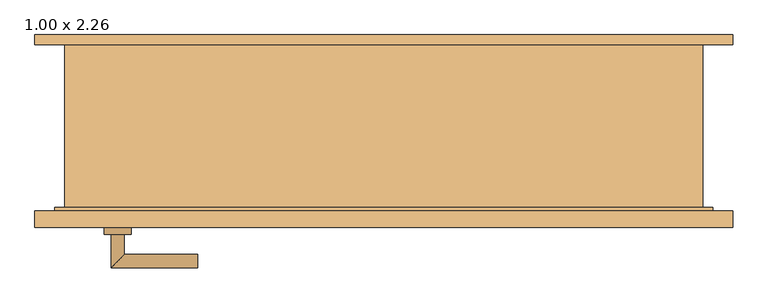
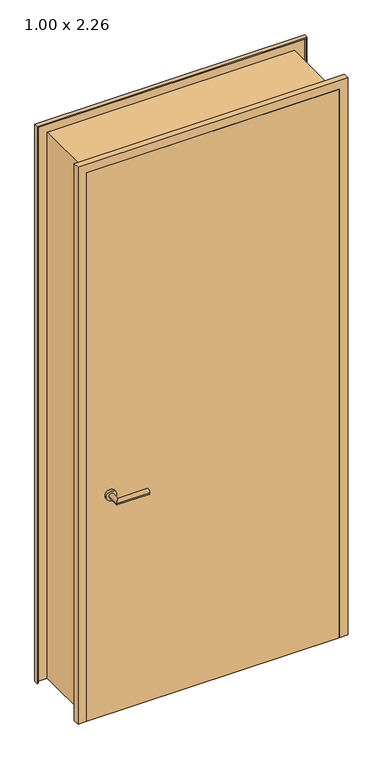
"""IFC4 building model written with IfcOpenShell, lengths in millimetres: door geometry, Drehflügel 1-flg - Stahlzarge : 1.00 x 2.26."""

import ifcopenshell
import ifcopenshell.guid

model = None  # the IFC model being written
_history = None  # IfcOwnerHistory: only IFC2X3 demands one
_inside = {}  # id of a spatial element -> (the spatial element, [elements in it])
_under = {}  # id of a project, library or spatial element -> (it, [spatial elements below it])
_declared = {}  # id of a project -> (the project, [libraries it declares])
_typed = {}  # id of a type object -> (the type object, [elements of that type])
_made_of = {}  # id of a material, layer set ... -> (it, [elements and type objects made of it])


def new_model(schema):
    """Start an empty IFC model of exactly this schema.

    Asked for "IFC4X3", IfcOpenShell would pick the latest addendum, in which some entities
    have other attributes; the version numbers below select the first issue.
    IFC2X3 requires an IfcOwnerHistory on every rooted entity: one is made here for all.
    """
    global model, _history
    if schema == "IFC4X3":
        model = ifcopenshell.file(schema_version=(4, 3, 0, 0))
    else:
        model = ifcopenshell.file(schema=schema)
    _inside.clear()
    _under.clear()
    _declared.clear()
    _typed.clear()
    _made_of.clear()
    _history = None
    if model.schema == "IFC2X3":
        org = make("IfcOrganization", Name="unknown")
        user = make(
            "IfcPersonAndOrganization",
            ThePerson=make("IfcPerson", FamilyName="unknown"),
            TheOrganization=org,
        )
        app = make(
            "IfcApplication",
            ApplicationDeveloper=org,
            Version="unknown",
            ApplicationFullName="unknown",
            ApplicationIdentifier="unknown",
        )
        _history = make(
            "IfcOwnerHistory",
            OwningUser=user,
            OwningApplication=app,
            ChangeAction="ADDED",
            CreationDate=0,
        )
    return model


def make(cls, **values):
    """One entity of the class cls with the attributes given. An attribute that is None is left unset."""
    return model.create_entity(
        cls, **{name: value for name, value in values.items() if value is not None}
    )


def rooted(cls, **values):
    """An entity with a GlobalId (a new one), such as an element, a storey or a relation."""
    return make(cls, GlobalId=ifcopenshell.guid.new(), OwnerHistory=_history, **values)


def si_unit(unit_type, name, prefix=None):
    """IfcSIUnit, for example si_unit("LENGTHUNIT", "METRE", prefix="MILLI")."""
    return make("IfcSIUnit", UnitType=unit_type, Prefix=prefix, Name=name)


def assignment(units):
    """IfcUnitAssignment: the units of a project."""
    return None if units is None else make("IfcUnitAssignment", Units=units)


def point(xyz):
    """IfcCartesianPoint."""
    return None if xyz is None else make("IfcCartesianPoint", Coordinates=xyz)


def direction(xyz):
    """IfcDirection."""
    return None if xyz is None else make("IfcDirection", DirectionRatios=xyz)


def frame(location, z_axis=None, x_axis=None):
    """IfcAxis2Placement3D, a coordinate frame: its origin and axes. An axis left out is left unset."""
    return make(
        "IfcAxis2Placement3D",
        Location=point(location),
        Axis=direction(z_axis),
        RefDirection=direction(x_axis),
    )


def frame_2d(location, x_axis=None):
    """IfcAxis2Placement2D, a coordinate frame in the plane: its origin and x axis."""
    return make(
        "IfcAxis2Placement2D", Location=point(location), RefDirection=direction(x_axis)
    )


def origin():
    """The frame at (0, 0, 0) with its axes left unset."""
    return frame((0.0, 0.0, 0.0))


def place(relative_to, where):
    """IfcLocalPlacement: puts the frame where relative to a parent placement (None: the world)."""
    return make(
        "IfcLocalPlacement", PlacementRelTo=relative_to, RelativePlacement=where
    )


def context(
    kind, dimensions, precision=None, world=None, true_north=None, identifier=None
):
    """IfcGeometricRepresentationContext, for example the 3D "Model" context."""
    return make(
        "IfcGeometricRepresentationContext",
        ContextIdentifier=identifier,
        ContextType=kind,
        CoordinateSpaceDimension=dimensions,
        Precision=precision,
        WorldCoordinateSystem=world,
        TrueNorth=true_north,
    )


def project(units=None, contexts=None):
    """IfcProject with its units and contexts."""
    return rooted(
        "IfcProject",
        Name="project",
        RepresentationContexts=contexts,
        UnitsInContext=assignment(units),
    )


def spatial(cls, under=None, at=None, **own):
    """A site, building, storey or space (cls), placed at a placement, below another one or the project."""
    s = rooted(cls, ObjectPlacement=at, **own)
    if under is not None:
        _under.setdefault(under.id(), (under, []))[1].append(s)
    return s


def polyline(points):
    """IfcPolyline through the points."""
    return make("IfcPolyline", Points=[point(p) for p in points])


def circle_curve(where, radius):
    """IfcCircle in the frame where."""
    return make("IfcCircle", Position=where, Radius=radius)


def ellipse_curve(where, semi_axis1, semi_axis2):
    """IfcEllipse in the frame where."""
    return make(
        "IfcEllipse", Position=where, SemiAxis1=semi_axis1, SemiAxis2=semi_axis2
    )


def trimmed(basis, trim1, trim2, sense, master):
    """IfcTrimmedCurve: the piece of a basis curve between two trims."""
    return make(
        "IfcTrimmedCurve",
        BasisCurve=basis,
        Trim1=trim1,
        Trim2=trim2,
        SenseAgreement=sense,
        MasterRepresentation=master,
    )


def segment(curve, same_sense, transition):
    """IfcCompositeCurveSegment."""
    return make(
        "IfcCompositeCurveSegment",
        Transition=transition,
        SameSense=same_sense,
        ParentCurve=curve,
    )


def composite_curve(segments, self_intersect=None):
    """IfcCompositeCurve: segments joined end to end."""
    return make("IfcCompositeCurve", Segments=segments, SelfIntersect=self_intersect)


def outline(outer, holes=None, kind="AREA"):
    """IfcArbitraryClosedProfileDef: a profile drawn as a closed curve; with holes, ...WithVoids."""
    if holes is None:
        return make("IfcArbitraryClosedProfileDef", ProfileType=kind, OuterCurve=outer)
    return make(
        "IfcArbitraryProfileDefWithVoids",
        ProfileType=kind,
        OuterCurve=outer,
        InnerCurves=holes,
    )


def extrude(swept, where, along, depth):
    """IfcExtrudedAreaSolid: the profile swept, set in the frame where, extruded along a direction by depth."""
    return make(
        "IfcExtrudedAreaSolid",
        SweptArea=swept,
        Position=where,
        ExtrudedDirection=direction(along),
        Depth=depth,
    )


def faces_of(points, faces, orient=None, outer=None):
    """IfcFace entities. A face is a list of loops; a loop is a list of indices into points, from 0.

    orient and outer hold one flag for each loop. By default every Orientation is true, the
    first loop of a face is its IfcFaceOuterBound and the others are IfcFaceBound.
    """
    made = []
    for i, loops in enumerate(faces):
        bounds = []
        for j, loop in enumerate(loops):
            is_outer = j == 0 if outer is None else outer[i][j]
            bounds.append(
                make(
                    "IfcFaceOuterBound" if is_outer else "IfcFaceBound",
                    Bound=make("IfcPolyLoop", Polygon=[points[k] for k in loop]),
                    Orientation=True if orient is None else orient[i][j],
                )
            )
        made.append(make("IfcFace", Bounds=bounds))
    return made


def faceted_brep(points, faces, orient=None, outer=None, voids=None):
    """IfcFacetedBrep: a solid bounded by flat faces; with voids (closed shells), ...WithVoids."""
    shared = [point(p) for p in points]
    hull = make("IfcClosedShell", CfsFaces=faces_of(shared, faces, orient, outer))
    if voids is None:
        return make("IfcFacetedBrep", Outer=hull)
    return make(
        "IfcFacetedBrepWithVoids",
        Outer=hull,
        Voids=[
            make(cls, CfsFaces=faces_of(shared, fs, o, b)) for cls, fs, o, b in voids
        ],
    )


def shape(context_of_items, identifier, shape_type, items):
    """IfcShapeRepresentation: the items that make up one representation, for example the "Body"."""
    return make(
        "IfcShapeRepresentation",
        ContextOfItems=context_of_items,
        RepresentationIdentifier=identifier,
        RepresentationType=shape_type,
        Items=items,
    )


def source(mapping_origin, context_of_items, identifier, shape_type, items):
    """IfcRepresentationMap: a shape defined once, which mapped items show again and again."""
    return make(
        "IfcRepresentationMap",
        MappingOrigin=mapping_origin,
        MappedRepresentation=shape(context_of_items, identifier, shape_type, items),
    )


def transform(
    local_origin,
    x_axis=None,
    y_axis=None,
    z_axis=None,
    scale=None,
    scale2=None,
    scale3=None,
    uniform=True,
):
    """IfcCartesianTransformationOperator3D, or its non-uniform kind. x_axis, y_axis, z_axis: its Axis1, 2, 3."""
    if uniform:
        return make(
            "IfcCartesianTransformationOperator3D",
            Axis1=direction(x_axis),
            Axis2=direction(y_axis),
            LocalOrigin=point(local_origin),
            Scale=scale,
            Axis3=direction(z_axis),
        )
    return make(
        "IfcCartesianTransformationOperator3DnonUniform",
        Axis1=direction(x_axis),
        Axis2=direction(y_axis),
        LocalOrigin=point(local_origin),
        Scale=scale,
        Axis3=direction(z_axis),
        Scale2=scale2,
        Scale3=scale3,
    )


def mapped(mapping_source, mapping_target):
    """IfcMappedItem: shows the shape of a source again, moved by a transform."""
    return make(
        "IfcMappedItem", MappingSource=mapping_source, MappingTarget=mapping_target
    )


def made_of(thing, what):
    """Note that an element or type object is made of a material, layer set ...; save() writes the relation."""
    if what is not None:
        _made_of.setdefault(what.id(), (what, []))[1].append(thing)
    return thing


def element(
    cls,
    number,
    at=None,
    inside=None,
    cuts=None,
    type_object=None,
    material=None,
    context=None,
    identifier="Body",
    shape_type=None,
    held_by="IfcProductDefinitionShape",
    body=None,
    shapes=None,
    **own,
):
    """One element of the class cls, such as IfcWall. Its Tag is "e" and its number.

    at: its placement. inside: the storey or other place that contains it. cuts: it is an
    opening in that element (IfcRelVoidsElement). A single representation is given by context,
    identifier, shape_type and body (its items); several are given by shapes. held_by: the class
    of the entity that holds the representations. save() writes the other relations.
    """
    e = rooted(cls, Tag="e%d" % number, ObjectPlacement=at, **own)
    if body is not None:
        shapes = [shape(context, identifier, shape_type, body)]
    if shapes is not None:
        e.Representation = make(held_by, Representations=shapes)
    if inside is not None:
        _inside.setdefault(inside.id(), (inside, []))[1].append(e)
    if cuts is not None:
        rooted(
            "IfcRelVoidsElement", RelatingBuildingElement=cuts, RelatedOpeningElement=e
        )
    if type_object is not None:
        _typed.setdefault(type_object.id(), (type_object, []))[1].append(e)
    return made_of(e, material)


def aggregate(whole, parts):
    """IfcRelAggregates: a whole, such as a stair, and the parts it consists of."""
    return rooted("IfcRelAggregates", RelatingObject=whole, RelatedObjects=parts)


def save(model, path):
    """Write the relations noted so far, then the file.

    IfcRelAggregates (storeys below a building ...), IfcRelContainedInSpatialStructure (elements
    in a storey), IfcRelDefinesByType, IfcRelAssociatesMaterial and IfcRelDeclares: one each for
    every whole, place, type object, material and project.
    """
    for whole, parts in _under.values():
        aggregate(whole, parts)
    for where, things in _inside.values():
        rooted(
            "IfcRelContainedInSpatialStructure",
            RelatedElements=things,
            RelatingStructure=where,
        )
    for kind, things in _typed.values():
        rooted("IfcRelDefinesByType", RelatedObjects=things, RelatingType=kind)
    for what, things in _made_of.values():
        rooted("IfcRelAssociatesMaterial", RelatedObjects=things, RelatingMaterial=what)
    for by, libraries in _declared.values():
        rooted("IfcRelDeclares", RelatingContext=by, RelatedDefinitions=libraries)
    model.write(path)


def plane_surface(at):
    """IfcPlane: the flat surface through the origin of the frame at, square to its z axis."""
    return make("IfcPlane", Position=at)


def cylinder_surface(at, radius):
    """IfcCylindricalSurface: all points at the distance radius from the z axis of the frame at."""
    return make("IfcCylindricalSurface", Position=at, Radius=radius)


def advanced_brep(points, edges, surfaces, faces):
    """IfcAdvancedBrep: a solid bounded by faces that lie on surfaces and meet in shared edges.

    An edge is (start, end): straight between two places in points (the first is 0);
    or (start, end, curve); or (start, end, curve, False) where it runs against its curve.
    A face is (place in surfaces, loops), or (place, loops, False) where it looks against
    its surface's normal. A loop lists edges by number (the first is 1), with a minus sign
    where the edge is run from its end to its start. The first loop is the outer one.
    """
    corners = [point(p) for p in points]
    vertices = [make("IfcVertexPoint", VertexGeometry=c) for c in corners]
    made = []
    for start, end, *more in edges:
        made.append(
            make(
                "IfcEdgeCurve",
                EdgeStart=vertices[start],
                EdgeEnd=vertices[end],
                EdgeGeometry=more[0] if more else make("IfcPolyline", Points=[corners[start], corners[end]]),
                SameSense=more[1] if len(more) > 1 else True,
            )
        )
    hull = []
    for where, loops, *sense in faces:
        bounds = []
        for j, loop in enumerate(loops):
            ring = [make("IfcOrientedEdge", EdgeElement=made[abs(k) - 1], Orientation=k > 0) for k in loop]
            bounds.append(
                make(
                    "IfcFaceOuterBound" if j == 0 else "IfcFaceBound",
                    Bound=make("IfcEdgeLoop", EdgeList=ring),
                    Orientation=True,
                )
            )
        hull.append(make("IfcAdvancedFace", Bounds=bounds, FaceSurface=surfaces[where], SameSense=sense[0] if sense else True))
    return make("IfcAdvancedBrep", Outer=make("IfcClosedShell", CfsFaces=hull))


def door_1_00_x_2_26_2441bcad(model_context):
    return source(origin(), model_context, "Body", "SolidModel", [
        advanced_brep(
        [(-410.0, -114.4346141, 1000.0), (-390.0, -114.4346141, 1000.0), (-390.0, -64.4346141, 1000.0), (-410.0, -44.4346141, 1000.0), (-280.0, -44.4346141, 1000.0), (-280.0, -64.4346141, 1000.0)],
        [
            (0, 1, circle_curve(frame((-400.0, -114.4346141, 1000.0), z_axis=(0.0, -1.0, 0.0), x_axis=(1.0, 0.0, 0.0)), 10.0)),
            (1, 0, circle_curve(frame((-400.0, -114.4346141, 1000.0), z_axis=(0.0, -1.0, 0.0), x_axis=(1.0, 0.0, 0.0)), 10.0)),
            (1, 2),
            (2, 3, ellipse_curve(frame((-400.0, -54.4346141, 1000.0), z_axis=(-0.7071067811865385, -0.7071067811865565, 0.0), x_axis=(0.7071067811865563, -0.7071067811865386, 0.0)), 14.1421356, 10.0)),
            (3, 0),
            (3, 2, ellipse_curve(frame((-400.0, -54.4346141, 1000.0), z_axis=(-0.7071067811865385, -0.7071067811865565, 0.0), x_axis=(0.7071067811865563, -0.7071067811865386, 0.0)), 14.1421356, 10.0)),
            (4, 5, circle_curve(frame((-280.0, -54.4346141, 1000.0), z_axis=(1.0, 0.0, 0.0), x_axis=(0.0, -1.0, 0.0)), 10.0)),
            (5, 4, circle_curve(frame((-280.0, -54.4346141, 1000.0), z_axis=(1.0, 0.0, 0.0), x_axis=(0.0, -1.0, 0.0)), 10.0)),
            (2, 5),
            (4, 3),
        ],
        [
            plane_surface(frame((-400.0, -114.4346141, -287.7526403), z_axis=(0.0, -1.0, 0.0), x_axis=(0.0, 0.0, 1.0))),
            cylinder_surface(frame((-400.0, -114.4346141, 1000.0), z_axis=(0.0, -1.0, 0.0), x_axis=(1.0, 0.0, 0.0)), 10.0),
            plane_surface(frame((-280.0, -54.4346141, -287.7526403), z_axis=(1.0, 0.0, 0.0), x_axis=(0.0, 0.0, 1.0))),
            cylinder_surface(frame((-400.0, -54.4346141, 1000.0), z_axis=(-1.0, 0.0, 0.0), x_axis=(0.0, -1.0, 0.0)), 10.0),
        ],
        [
            (0, [[1, 2]]),
            (1, [[3, 4, 5, -2]]),
            (1, [[-5, 6, -3, -1]]),
            (2, [[7, 8]]),
            (3, [[9, -7, 10, -4]]),
            (3, [[-10, -8, -9, -6]]),
        ],
    ),
        advanced_brep(
        [(-390.0, -174.4346141, 1000.0), (-410.0, -174.4346141, 1000.0), (-410.0, -224.4346141, 1000.0), (-390.0, -204.4346141, 1000.0), (-280.0, -204.4346141, 1000.0), (-280.0, -224.4346141, 1000.0)],
        [
            (0, 1, circle_curve(frame((-400.0, -174.4346141, 1000.0), z_axis=(0.0, 1.0, 0.0), x_axis=(-1.0, 0.0, 0.0)), 10.0)),
            (1, 0, circle_curve(frame((-400.0, -174.4346141, 1000.0), z_axis=(0.0, 1.0, 0.0), x_axis=(-1.0, 0.0, 0.0)), 10.0)),
            (1, 2),
            (2, 3, ellipse_curve(frame((-400.0, -214.4346141, 1000.0), z_axis=(-0.7071067811865475, 0.7071067811865475, 0.0), x_axis=(0.7071067811865474, 0.7071067811865476, 0.0)), 14.1421356, 10.0)),
            (3, 0),
            (3, 2, ellipse_curve(frame((-400.0, -214.4346141, 1000.0), z_axis=(-0.7071067811865475, 0.7071067811865475, 0.0), x_axis=(0.7071067811865474, 0.7071067811865476, 0.0)), 14.1421356, 10.0)),
            (4, 5, circle_curve(frame((-280.0, -214.4346141, 1000.0), z_axis=(1.0, 0.0, 0.0), x_axis=(0.0, -1.0, 0.0)), 10.0)),
            (5, 4, circle_curve(frame((-280.0, -214.4346141, 1000.0), z_axis=(1.0, 0.0, 0.0), x_axis=(0.0, -1.0, 0.0)), 10.0)),
            (2, 5),
            (4, 3),
        ],
        [
            plane_surface(frame((-400.0, -174.4346141, -287.7526403), z_axis=(0.0, 1.0, 0.0), x_axis=(0.0, 0.0, 1.0))),
            cylinder_surface(frame((-400.0, -174.4346141, 1000.0), z_axis=(0.0, 1.0, 0.0), x_axis=(-1.0, 0.0, 0.0)), 10.0),
            plane_surface(frame((-280.0, -214.4346141, -287.7526403), z_axis=(1.0, 0.0, 0.0), x_axis=(0.0, 0.0, 1.0))),
            cylinder_surface(frame((-400.0, -214.4346141, 1000.0), z_axis=(-1.0, 0.0, 0.0), x_axis=(0.0, -1.0, 0.0)), 10.0),
        ],
        [
            (0, [[1, 2]]),
            (1, [[3, 4, 5, -2]]),
            (1, [[-5, 6, -3, -1]]),
            (2, [[7, 8]]),
            (3, [[9, -7, 10, -4]]),
            (3, [[-10, -8, -9, -6]]),
        ],
    ),
        extrude(outline(composite_curve([segment(trimmed(circle_curve(frame_2d((1000.0, -400.0)), 20.0), [point((1000.0, -420.0))], [point((1000.0, -380.0))], False, "CARTESIAN"), True, "CONTINUOUS"), segment(trimmed(circle_curve(frame_2d((1000.0, -400.0)), 20.0), [point((1000.0, -380.0))], [point((1000.0, -420.0))], False, "CARTESIAN"), True, "CONTINUOUS")], self_intersect=False)), frame((0.0, -114.4346141, 0.0), z_axis=(0.0, 1.0, 0.0), x_axis=(0.0, 0.0, 1.0)), (0.0, 0.0, 1.0), 10.0),
        extrude(outline(composite_curve([segment(trimmed(circle_curve(frame_2d((1000.0, -400.0)), 20.0), [point((1000.0, -420.0))], [point((1000.0, -380.0))], False, "CARTESIAN"), True, "CONTINUOUS"), segment(trimmed(circle_curve(frame_2d((1000.0, -400.0)), 20.0), [point((1000.0, -380.0))], [point((1000.0, -420.0))], False, "CARTESIAN"), True, "CONTINUOUS")], self_intersect=False)), frame((0.0, -174.4346141, 0.0), z_axis=(0.0, 1.0, 0.0), x_axis=(0.0, 0.0, 1.0)), (0.0, 0.0, 1.0), 10.0),
        extrude(outline(polyline([(490.0, -139.4346141), (490.0, -164.4346141), (-490.0, -164.4346141), (-490.0, -139.4346141), (490.0, -139.4346141)])), frame((0.0, 0.0, 100.0), z_axis=(0.0, 0.0, 1.0), x_axis=(1.0, 0.0, 0.0)), (0.0, 0.0, 1.0), 2250.0),
        faceted_brep([(524.4603207, 125.5653859, 100.0), (524.4603207, 110.5653859, 100.0), (519.4603207, 110.5653859, 100.0), (519.4603207, 120.5653859, 100.0), (480.0, 120.5653859, 100.0), (480.0, -134.4346141, 100.0), (495.0, -134.4346141, 100.0), (495.0, -159.4346141, 100.0), (519.4603207, -159.4346141, 100.0), (519.4603207, -139.4346141, 100.0), (524.4603207, -139.4346141, 100.0), (524.4603207, -164.4346141, 100.0), (490.0, -164.4346141, 100.0), (490.0, -139.4346141, 100.0), (475.0, -139.4346141, 100.0), (475.0, 125.5653859, 100.0), (475.0, 125.5653859, 2335.0), (-475.0, 125.5653859, 2335.0), (-475.0, 125.5653859, 100.0), (-524.4603207, 125.5653859, 100.0), (-524.4603207, 125.5653859, 2384.4603207), (524.4603207, 125.5653859, 2384.4603207), (475.0, -139.4346141, 2335.0), (490.0, -139.4346141, 2350.0), (-490.0, -139.4346141, 2350.0), (-490.0, -139.4346141, 100.0), (-475.0, -139.4346141, 100.0), (-475.0, -139.4346141, 2335.0), (490.0, -164.4346141, 2350.0), (524.4603207, -164.4346141, 2384.4603207), (-524.4603207, -164.4346141, 2384.4603207), (-524.4603207, -164.4346141, 100.0), (-490.0, -164.4346141, 100.0), (-490.0, -164.4346141, 2350.0), (524.4603207, -139.4346141, 2384.4603207), (519.4603207, -139.4346141, 2379.4603207), (-519.4603207, -139.4346141, 2379.4603207), (-519.4603207, -139.4346141, 100.0), (-524.4603207, -139.4346141, 100.0), (-524.4603207, -139.4346141, 2384.4603207), (519.4603207, -159.4346141, 2379.4603207), (495.0, -159.4346141, 2355.0), (-495.0, -159.4346141, 2355.0), (-495.0, -159.4346141, 100.0), (-519.4603207, -159.4346141, 100.0), (-519.4603207, -159.4346141, 2379.4603207), (495.0, -134.4346141, 2355.0), (480.0, -134.4346141, 2340.0), (-480.0, -134.4346141, 2340.0), (-480.0, -134.4346141, 100.0), (-495.0, -134.4346141, 100.0), (-495.0, -134.4346141, 2355.0), (480.0, 120.5653859, 2340.0), (519.4603207, 120.5653859, 2379.4603207), (-519.4603207, 120.5653859, 2379.4603207), (-519.4603207, 120.5653859, 100.0), (-480.0, 120.5653859, 100.0), (-480.0, 120.5653859, 2340.0), (519.4603207, 110.5653859, 2379.4603207), (524.4603207, 110.5653859, 2384.4603207), (-524.4603207, 110.5653859, 2384.4603207), (-524.4603207, 110.5653859, 100.0), (-519.4603207, 110.5653859, 100.0), (-519.4603207, 110.5653859, 2379.4603207)], [[[0, 1, 2, 3, 4, 5, 6, 7, 8, 9, 10, 11, 12, 13, 14, 15]], [[15, 16, 17, 18, 19, 20, 21, 0]], [[14, 22, 16, 15]], [[13, 23, 24, 25, 26, 27, 22, 14]], [[12, 28, 23, 13]], [[11, 29, 30, 31, 32, 33, 28, 12]], [[10, 34, 29, 11]], [[9, 35, 36, 37, 38, 39, 34, 10]], [[8, 40, 35, 9]], [[7, 41, 42, 43, 44, 45, 40, 8]], [[6, 46, 41, 7]], [[5, 47, 48, 49, 50, 51, 46, 6]], [[4, 52, 47, 5]], [[3, 53, 54, 55, 56, 57, 52, 4]], [[2, 58, 53, 3]], [[1, 59, 60, 61, 62, 63, 58, 2]], [[0, 21, 59, 1]], [[20, 19, 61, 60]], [[19, 18, 26, 25, 32, 31, 38, 37, 44, 43, 50, 49, 56, 55, 62, 61]], [[27, 26, 18, 17]], [[33, 32, 25, 24]], [[39, 38, 31, 30]], [[45, 44, 37, 36]], [[51, 50, 43, 42]], [[57, 56, 49, 48]], [[63, 62, 55, 54]], [[22, 27, 17, 16]], [[28, 33, 24, 23]], [[34, 39, 30, 29]], [[40, 45, 36, 35]], [[46, 51, 42, 41]], [[52, 57, 48, 47]], [[58, 63, 54, 53]], [[21, 20, 60, 59]]]),
    ])


if __name__ == "__main__":
    model = new_model("IFC4")
    model_context = context("Model", 3, world=origin())
    ifc_project = project(units=[si_unit("LENGTHUNIT", "METRE", prefix="MILLI")], contexts=[model_context])
    site = spatial("IfcSite", under=ifc_project)
    building = spatial("IfcBuilding", under=site)
    placement = place(None, origin())
    door_1_00_x_2_26_shape = door_1_00_x_2_26_2441bcad(model_context)
    element("IfcDoor", 1, ObjectType="Drehflügel 1-flg - Stahlzarge : 1.00 x 2.26", at=placement, inside=building, context=model_context, shape_type="MappedRepresentation", body=[
        mapped(door_1_00_x_2_26_shape, transform((0.0, 0.0, 0.0), x_axis=(1.0, 0.0, 0.0), y_axis=(0.0, 1.0, 0.0), z_axis=(0.0, 0.0, 1.0))),
    ])
    save(model, "model.ifc")

# Revit data of these elements
# Type "Drehflügel 1-flg - Stahlzarge : 1.00 x 2.26"
#   Construction Type Id = "MDOOR"
#   Type Mark = "20"
#   Operation = "SingleSwingRight"
#   Keynote = "16.03"
#   Analytic Construction = "Metall"
#   Thermal Resistance (R) = 0.270117 (m²·K)/W
#   Heat Transfer Coefficient (U) = 3.7021 W/(m²·K)
#   Rough Width = 1.000 m
#   Rough Height [instance default] = 2.360 m
#   Höhe Türgriff [instance default] = 0.900 m
#   Height = 2.260 m
#   Fußbodenaufbau [instance default] = 0.100 m
#   Width = 1.000 m
#   Sichtbarkeit Sturzlinien [instance default] = yes
#   Türgriff auswählen [instance default] = element 221079
#   Türgriff [instance default] = none
#   Türflügel [instance default] = none
#   Rahmen/Pfosten [instance default] = Metall - Lackiert - Grau
#   Visual Light Transmittance = 0
#   Solar Heat Gain Coefficient = 0
#   Function = (empty or 0)
#   Wall Closure = (empty or 0)
# Element 1 (IfcDoor, "Drehflügel 1-flg - Stahlzarge : 1.00 x 2.26")
#   Materials on its faces: "Metall - Lackiert - Grau", "Metall - Chrom", "Holz - Birke"
# Materials
#   "Metall - Lackiert - Grau": class "Farbe 1", colour RGB 98 98 98, transparency 0, Cost = 0
#   "Metall - Chrom": class "Metall", colour RGB 247 247 247, transparency 0, Cost = 0
#   "Holz - Birke": class "Holz", colour RGB 213 164 103, transparency 0, Cost = 0
